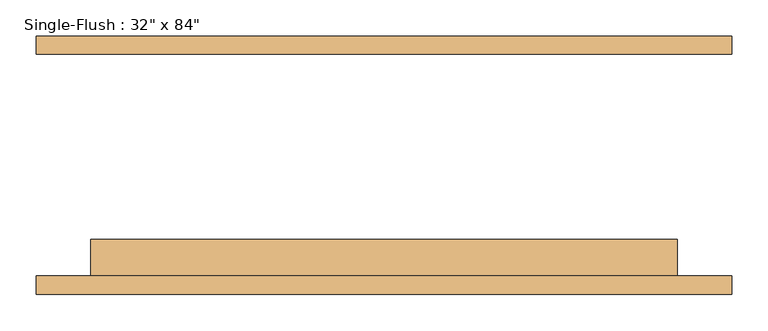
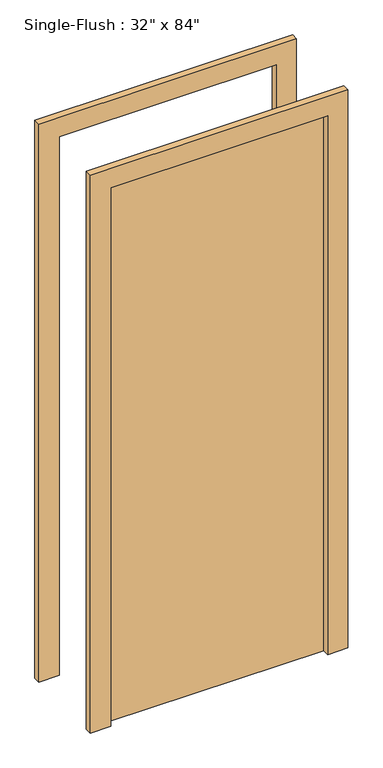
"""IFC4 building model written with IfcOpenShell, lengths in millimetres: door geometry."""

from ifc_helpers import new_model, si_unit, frame, origin, origin_with_axes, place, context, project, spatial, polyline, outline, extrude, source, transform, mapped, element, save


def door_7d01847f(model_context):
    return source(origin(), model_context, "Body", "SweptSolid", [
        extrude(outline(polyline([(2209.8, -482.6), (0.0, -482.6), (0.0, -406.4), (2133.6, -406.4), (2133.6, 406.4), (0.0, 406.4), (0.0, 482.6), (2209.8, 482.6), (2209.8, -482.6)])), frame((0.0, -179.3875, 0.0), z_axis=(0.0, 1.0, 0.0), x_axis=(0.0, 0.0, 1.0)), (0.0, 0.0, 1.0), 25.4),
        extrude(outline(polyline([(2209.8, 482.6), (2209.8, -482.6), (0.0, -482.6), (0.0, -406.4), (2133.6, -406.4), (2133.6, 406.4), (0.0, 406.4), (0.0, 482.6), (2209.8, 482.6)])), frame((0.0, 153.9875, 0.0), z_axis=(0.0, 1.0, 0.0), x_axis=(0.0, 0.0, 1.0)), (0.0, 0.0, 1.0), 25.4),
        extrude(outline(polyline([(406.4, -103.1875), (406.4, -153.9875), (-406.4, -153.9875), (-406.4, -103.1875), (406.4, -103.1875)])), origin_with_axes(), (0.0, 0.0, 1.0), 2133.6),
    ])


if __name__ == "__main__":
    model = new_model("IFC4")
    model_context = context("Model", 3, world=origin())
    ifc_project = project(units=[si_unit("LENGTHUNIT", "METRE", prefix="MILLI")], contexts=[model_context])
    site = spatial("IfcSite", under=ifc_project)
    building = spatial("IfcBuilding", under=site)
    placement = place(None, origin())
    door_shape = door_7d01847f(model_context)
    element("IfcDoor", 1, ObjectType="Single-Flush : 32\" x 84\"", at=placement, inside=building, context=model_context, shape_type="MappedRepresentation", body=[
        mapped(door_shape, transform((0.0, 0.0, 0.0), x_axis=(1.0, 0.0, 0.0), y_axis=(0.0, 1.0, 0.0), z_axis=(0.0, 0.0, 1.0))),
    ])
    save(model, "model.ifc")

# Revit data of these elements
# Type "Single-Flush : 32\" x 84\""
#   Type Mark = "10"
#   Construction Type Id = "MDOOR"
#   Assembly Code = "C1020"
#   Analytic Construction = "Metal"
#   Thickness = 0' - 2"
#   Heat Transfer Coefficient (U) = 3.7021 W/(m²·K)
#   Height = 7' - 0"
#   Trim Projection Ext = 0' - 1"
#   Trim Projection Int = 0' - 1"
#   Trim Width = 0' - 3"
#   Width = 2' - 8"
#   Door Material = Door - Panel
#   Frame Material = Door - Frame
#   Visual Light Transmittance = 0
#   Solar Heat Gain Coefficient = 0
#   Function = (empty or 0)
#   Wall Closure = (empty or 0)
# Element 1 (IfcDoor, "Single-Flush : 32\" x 84\"")
#   Materials on its faces: "Door - Frame", "Door - Panel"
# Materials
#   "Door - Panel": class "Wood", colour RGB 210 159 95, transparency 0
#   "Door - Frame": class "Miscellaneous", colour RGB 118 70 51, transparency 0
